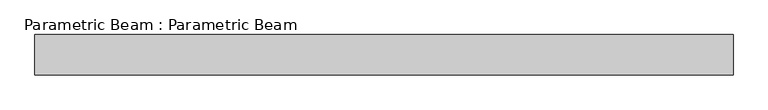
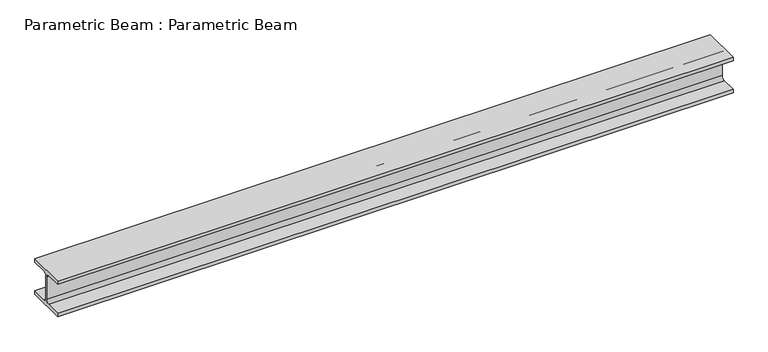
"""IFC4 building model written with IfcOpenShell, lengths in millimetres: beam geometry, Parametric Beam : Parametric Beam."""

from ifc_helpers import new_model, si_unit, point, frame, frame_2d, origin, place, context, project, spatial, polyline, circle_curve, trimmed, segment, composite_curve, outline, extrude, source, transform, mapped, element, save


def parametric_beam_parametric_beam_d4aa52de(model_context):
    return source(origin(), model_context, "Body", "SweptSolid", [
        extrude(outline(composite_curve([segment(polyline([(3.75, 72.0), (3.75, -72.0)]), True, "CONTINUOUS"), segment(trimmed(circle_curve(frame_2d((24.75, -72.0)), 21.0), [point((3.75, -72.0))], [point((24.75, -93.0))], True, "CARTESIAN"), True, "CONTINUOUS"), segment(polyline([(24.75, -93.0), (120.0, -93.0), (120.0, -115.0), (-120.0, -115.0), (-120.0, -93.0), (-24.75, -93.0)]), True, "CONTINUOUS"), segment(trimmed(circle_curve(frame_2d((-24.75, -72.0)), 21.0), [point((-24.75, -93.0))], [point((-3.75, -72.0))], True, "CARTESIAN"), True, "CONTINUOUS"), segment(polyline([(-3.75, -72.0), (-3.75, 72.0)]), True, "CONTINUOUS"), segment(trimmed(circle_curve(frame_2d((-24.75, 72.0)), 21.0), [point((-3.75, 72.0))], [point((-24.75, 93.0))], True, "CARTESIAN"), True, "CONTINUOUS"), segment(polyline([(-24.75, 93.0), (-120.0, 93.0), (-120.0, 115.0), (120.0, 115.0), (120.0, 93.0), (24.75, 93.0)]), True, "CONTINUOUS"), segment(trimmed(circle_curve(frame_2d((24.75, 72.0)), 21.0), [point((24.75, 93.0))], [point((3.75, 72.0))], True, "CARTESIAN"), True, "CONTINUOUS")], self_intersect=False)), frame((-2069.946659, 0.0, 0.0), z_axis=(1.0, 0.0, 0.0), x_axis=(0.0, 1.0, 0.0)), (0.0, 0.0, 1.0), 4139.893318),
    ])


if __name__ == "__main__":
    model = new_model("IFC4")
    model_context = context("Model", 3, world=origin())
    ifc_project = project(units=[si_unit("LENGTHUNIT", "METRE", prefix="MILLI")], contexts=[model_context])
    site = spatial("IfcSite", under=ifc_project)
    building = spatial("IfcBuilding", under=site)
    placement = place(None, origin())
    parametric_beam_parametric_beam_shape = parametric_beam_parametric_beam_d4aa52de(model_context)
    element("IfcBeam", 1, ObjectType="Parametric Beam : Parametric Beam", at=placement, inside=building, context=model_context, shape_type="MappedRepresentation", body=[
        mapped(parametric_beam_parametric_beam_shape, transform((0.0, 0.0, 0.0), x_axis=(1.0, 0.0, 0.0), y_axis=(0.0, 1.0, 0.0), z_axis=(0.0, 0.0, 1.0))),
    ])
    save(model, "model.ifc")

# Revit data of these elements
# Type "Parametric Beam : Parametric Beam"
#   MHP_PRO_Name [instance default] = "HEA"
#   r [instance default] = 0.021 m
#   h [instance default] = 0.3 m
#   b [instance default] = 0.24 m
#   Tw [instance default] = 0.0075 m
#   Tf [instance default] = 0.012 m
#   Length [instance default] = 3 m
#   Viktor_Change [instance default] = yes
# Element 1 (IfcBeam, "Parametric Beam : Parametric Beam")
#   MHP_PRO_Name = "HEA240"
#   h = 0.23 m
#   Tf = 0.022 m
#   Viktor_Change = no
